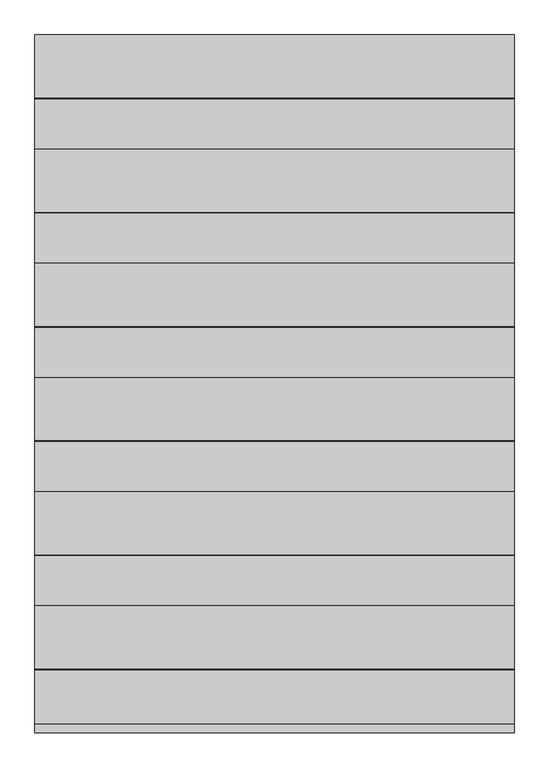
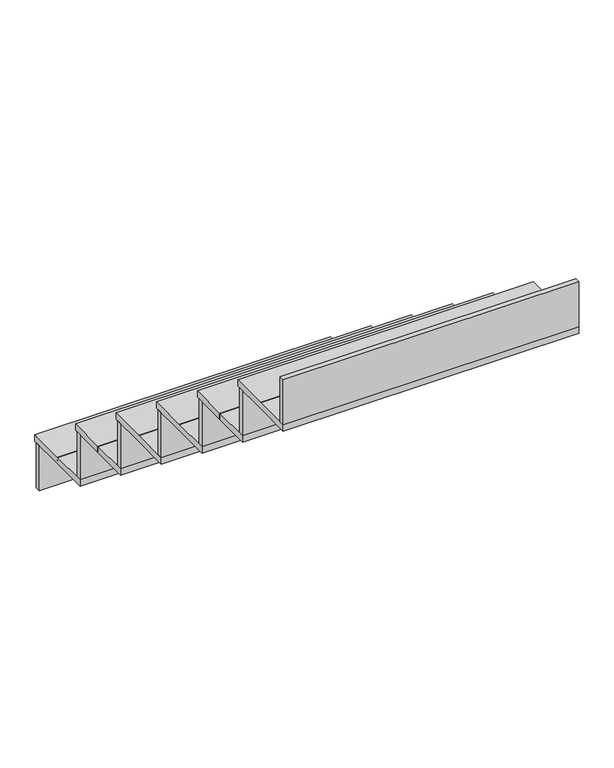
"""IFC4 building model written with IfcOpenShell, lengths in millimetres: stair flight geometry."""

from ifc_helpers import new_model, si_unit, frame, origin, place, context, project, spatial, polyline, outline, extrude, source, transform, mapped, element, save


def stair_flight_755c3211(model_context):
    return source(origin(), model_context, "Body", "SweptSolid", [
        extrude(outline(polyline([(-23943.9164763, -9473.4570712), (-23943.9164763, -9454.4070712), (-22877.1164763, -9454.4070712), (-22877.1164763, -9473.4570712), (-23943.9164763, -9473.4570712)])), frame((0.0, 0.0, 1371.6), z_axis=(0.0, 0.0, 1.0), x_axis=(1.0, 0.0, 0.0)), (0.0, 0.0, 1.0), 172.0311384),
        extrude(outline(polyline([(-9584.5820712, 1543.6311384), (-9584.5820712, 1555.3854105), (-9587.7570712, 1555.3854105), (-9587.7570712, 1543.6311384), (-9727.4570712, 1543.6311384), (-9727.4570712, 1567.5428571), (-9587.7570712, 1567.5428571), (-9587.7570712, 1555.7885851), (-9584.5820712, 1555.7885851), (-9584.5820712, 1567.5428571), (-9444.8820712, 1567.5428571), (-9444.8820712, 1543.6311384), (-9584.5820712, 1543.6311384)])), frame((-23943.9164763, 0.0, 0.0), z_axis=(1.0, 0.0, 0.0), x_axis=(0.0, 1.0, 0.0)), (0.0, 0.0, 1.0), 1066.8),
        extrude(outline(polyline([(-23943.9164763, -9727.4570712), (-23943.9164763, -9708.4070712), (-22877.1164763, -9708.4070712), (-22877.1164763, -9727.4570712), (-23943.9164763, -9727.4570712)])), frame((0.0, 0.0, 1567.5428571), z_axis=(0.0, 0.0, 1.0), x_axis=(1.0, 0.0, 0.0)), (0.0, 0.0, 1.0), 172.0311384),
        extrude(outline(polyline([(-9838.5820712, 1739.5739955), (-9838.5820712, 1751.3282676), (-9841.7570712, 1751.3282676), (-9841.7570712, 1739.5739955), (-9981.4570712, 1739.5739955), (-9981.4570712, 1763.4857143), (-9841.7570712, 1763.4857143), (-9841.7570712, 1751.7314422), (-9838.5820712, 1751.7314422), (-9838.5820712, 1763.4857143), (-9698.8820712, 1763.4857143), (-9698.8820712, 1739.5739955), (-9838.5820712, 1739.5739955)])), frame((-23943.9164763, 0.0, 0.0), z_axis=(1.0, 0.0, 0.0), x_axis=(0.0, 1.0, 0.0)), (0.0, 0.0, 1.0), 1066.8),
        extrude(outline(polyline([(-23943.9164763, -9981.4570712), (-23943.9164763, -9962.4070712), (-22877.1164763, -9962.4070712), (-22877.1164763, -9981.4570712), (-23943.9164763, -9981.4570712)])), frame((0.0, 0.0, 1763.4857143), z_axis=(0.0, 0.0, 1.0), x_axis=(1.0, 0.0, 0.0)), (0.0, 0.0, 1.0), 172.0311384),
        extrude(outline(polyline([(-10092.5820712, 1935.5168527), (-10092.5820712, 1947.2711248), (-10095.7570712, 1947.2711248), (-10095.7570712, 1935.5168527), (-10235.4570712, 1935.5168527), (-10235.4570712, 1959.4285714), (-10095.7570712, 1959.4285714), (-10095.7570712, 1947.6742994), (-10092.5820712, 1947.6742994), (-10092.5820712, 1959.4285714), (-9952.8820712, 1959.4285714), (-9952.8820712, 1935.5168527), (-10092.5820712, 1935.5168527)])), frame((-23943.9164763, 0.0, 0.0), z_axis=(1.0, 0.0, 0.0), x_axis=(0.0, 1.0, 0.0)), (0.0, 0.0, 1.0), 1066.8),
        extrude(outline(polyline([(-23943.9164763, -10235.4570712), (-23943.9164763, -10216.4070712), (-22877.1164763, -10216.4070712), (-22877.1164763, -10235.4570712), (-23943.9164763, -10235.4570712)])), frame((0.0, 0.0, 1959.4285714), z_axis=(0.0, 0.0, 1.0), x_axis=(1.0, 0.0, 0.0)), (0.0, 0.0, 1.0), 172.0311384),
        extrude(outline(polyline([(-10346.5820712, 2131.4597098), (-10346.5820712, 2143.2139819), (-10349.7570712, 2143.2139819), (-10349.7570712, 2131.4597098), (-10489.4570712, 2131.4597098), (-10489.4570712, 2155.3714286), (-10349.7570712, 2155.3714286), (-10349.7570712, 2143.6171565), (-10346.5820712, 2143.6171565), (-10346.5820712, 2155.3714286), (-10206.8820712, 2155.3714286), (-10206.8820712, 2131.4597098), (-10346.5820712, 2131.4597098)])), frame((-23943.9164763, 0.0, 0.0), z_axis=(1.0, 0.0, 0.0), x_axis=(0.0, 1.0, 0.0)), (0.0, 0.0, 1.0), 1066.8),
        extrude(outline(polyline([(-23943.9164763, -10489.4570712), (-23943.9164763, -10470.4070712), (-22877.1164763, -10470.4070712), (-22877.1164763, -10489.4570712), (-23943.9164763, -10489.4570712)])), frame((0.0, 0.0, 2155.3714286), z_axis=(0.0, 0.0, 1.0), x_axis=(1.0, 0.0, 0.0)), (0.0, 0.0, 1.0), 172.0311384),
        extrude(outline(polyline([(-10600.5820712, 2327.402567), (-10600.5820712, 2339.156839), (-10603.7570712, 2339.156839), (-10603.7570712, 2327.402567), (-10743.4570712, 2327.402567), (-10743.4570712, 2351.3142857), (-10603.7570712, 2351.3142857), (-10603.7570712, 2339.5600136), (-10600.5820712, 2339.5600136), (-10600.5820712, 2351.3142857), (-10460.8820712, 2351.3142857), (-10460.8820712, 2327.402567), (-10600.5820712, 2327.402567)])), frame((-23943.9164763, 0.0, 0.0), z_axis=(1.0, 0.0, 0.0), x_axis=(0.0, 1.0, 0.0)), (0.0, 0.0, 1.0), 1066.8),
        extrude(outline(polyline([(-23943.9164763, -10743.4570712), (-23943.9164763, -10724.4070712), (-22877.1164763, -10724.4070712), (-22877.1164763, -10743.4570712), (-23943.9164763, -10743.4570712)])), frame((0.0, 0.0, 2351.3142857), z_axis=(0.0, 0.0, 1.0), x_axis=(1.0, 0.0, 0.0)), (0.0, 0.0, 1.0), 172.0311384),
        extrude(outline(polyline([(-23943.9164763, -10997.4570712), (-23943.9164763, -10978.4070712), (-22877.1164763, -10978.4070712), (-22877.1164763, -10997.4570712), (-23943.9164763, -10997.4570712)])), frame((0.0, 0.0, 2547.2571429), z_axis=(0.0, 0.0, 1.0), x_axis=(1.0, 0.0, 0.0)), (0.0, 0.0, 1.0), 172.0311384),
        extrude(outline(polyline([(-10854.5820712, 2523.3454241), (-10854.5820712, 2535.0996962), (-10857.7570712, 2535.0996962), (-10857.7570712, 2523.3454241), (-10997.4570712, 2523.3454241), (-10997.4570712, 2547.2571429), (-10857.7570712, 2547.2571429), (-10857.7570712, 2535.5028708), (-10854.5820712, 2535.5028708), (-10854.5820712, 2547.2571429), (-10714.8820712, 2547.2571429), (-10714.8820712, 2523.3454241), (-10854.5820712, 2523.3454241)])), frame((-23943.9164763, 0.0, 0.0), z_axis=(1.0, 0.0, 0.0), x_axis=(0.0, 1.0, 0.0)), (0.0, 0.0, 1.0), 1066.8),
    ])


if __name__ == "__main__":
    model = new_model("IFC4")
    model_context = context("Model", 3, world=origin())
    ifc_project = project(units=[si_unit("LENGTHUNIT", "METRE", prefix="MILLI")], contexts=[model_context])
    site = spatial("IfcSite", under=ifc_project)
    building = spatial("IfcBuilding", under=site)
    placement = place(None, origin())
    stair_flight_shape = stair_flight_755c3211(model_context)
    element("IfcStairFlight", 1, at=placement, inside=building, context=model_context, shape_type="MappedRepresentation", body=[
        mapped(stair_flight_shape, transform((0.0, 0.0, 0.0), x_axis=(1.0, 0.0, 0.0), y_axis=(0.0, 1.0, 0.0), z_axis=(0.0, 0.0, 1.0))),
    ])
    save(model, "model.ifc")

# Revit data of these elements
# Element 1 (IfcStairFlight)
#   Materials on its faces: "Composite Deck - Trex - Select - 1x6 Square Edge Board - Saddle - 20'"
# Materials
#   "Composite Deck - Trex - Select - 1x6 Square Edge Board - Saddle - 20'": class "Wood", colour RGB 120 75 45, transparency 0, Keynote = "06 11 00", Model = "Trex Select® Composite Deck 1\" Square Edge Board", Manufacturer = "Trex", URL = "http://www.trex.com/", Description = "1x6 Trex Select® Composite Deck Square Edge Board", Cost = 0
